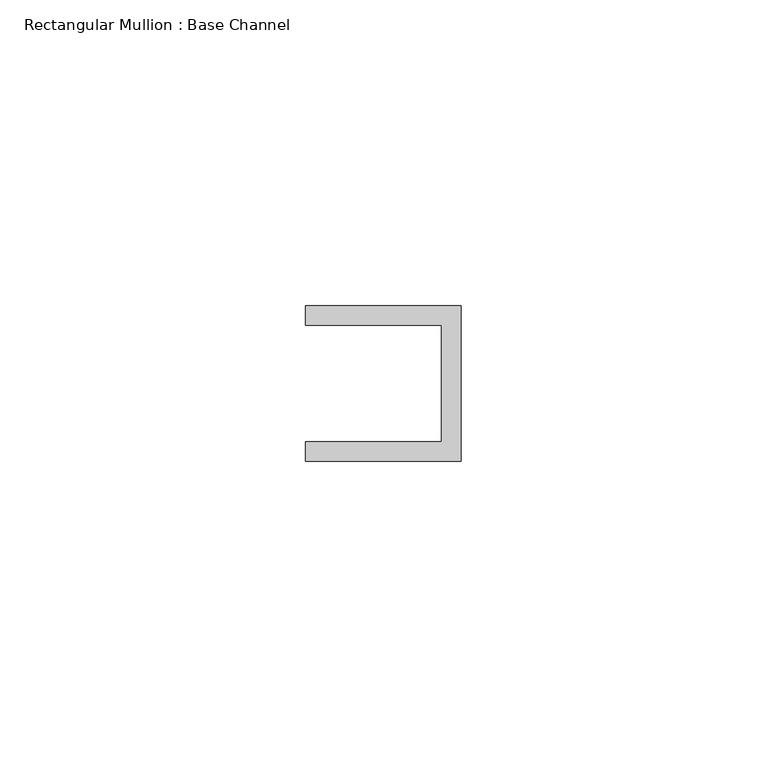
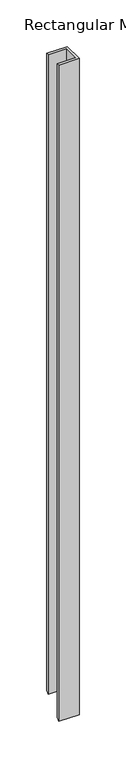
"""IFC4 building model written with IfcOpenShell, lengths in millimetres: member geometry, Rectangular Mullion : Base Channel."""

from ifc_helpers import new_model, si_unit, origin, place, context, project, spatial, faceted_brep, source, transform, mapped, element, save


def rectangular_mullion_base_channel_0fe43352(model_context):
    return source(origin(), model_context, "Body", "Brep", [
        faceted_brep([(0.0, -12.7, 0.0), (0.0, 12.7, 0.0), (-25.4, 12.7, 0.0), (-25.4, 9.525, 0.0), (-3.175, 9.525, 0.0), (-3.175, -9.525, 0.0), (-25.4, -9.525, 0.0), (-25.4, -12.7, 0.0), (0.0, -12.7, -858.1185498), (0.0, 12.7, -832.7185498), (-25.4, 12.7, -832.7185498), (-25.4, 9.525, -835.8935498), (-3.175, 9.525, -835.8935498), (-3.175, -9.525, -854.9435498), (-25.4, -9.525, -854.9435498), (-25.4, -12.7, -858.1185498)], [[[0, 1, 2, 3, 4, 5, 6, 7]], [[1, 0, 8, 9]], [[2, 1, 9, 10]], [[3, 2, 10, 11]], [[4, 3, 11, 12]], [[5, 4, 12, 13]], [[6, 5, 13, 14]], [[7, 6, 14, 15]], [[0, 7, 15, 8]], [[8, 15, 14, 13, 12, 11, 10, 9]]]),
    ])


if __name__ == "__main__":
    model = new_model("IFC4")
    model_context = context("Model", 3, world=origin())
    ifc_project = project(units=[si_unit("LENGTHUNIT", "METRE", prefix="MILLI")], contexts=[model_context])
    site = spatial("IfcSite", under=ifc_project)
    building = spatial("IfcBuilding", under=site)
    placement = place(None, origin())
    rectangular_mullion_base_channel_shape = rectangular_mullion_base_channel_0fe43352(model_context)
    element("IfcMember", 1, ObjectType="Rectangular Mullion : Base Channel", at=placement, inside=building, context=model_context, shape_type="MappedRepresentation", body=[
        mapped(rectangular_mullion_base_channel_shape, transform((0.0, 0.0, 0.0), x_axis=(1.0, 0.0, 0.0), y_axis=(0.0, 1.0, 0.0), z_axis=(0.0, 0.0, 1.0))),
    ])
    save(model, "model.ifc")

# Revit data of these elements
# Type "Rectangular Mullion : Base Channel"
#   built-in parameter 1007322 = 0.0833333 (stored number, unit not read)
#   built-in parameter 1007321 = 0.0416667 (stored number, unit not read)
#   built-in parameter 1007320 = -0.03125 (stored number, unit not read)
# Element 1 (IfcMember, "Rectangular Mullion : Base Channel")
#   Materials on its faces: "ALUM"
# Materials
#   "ALUM": class "Generic", colour RGB 157 157 157, transparency 0, Cost = 0
